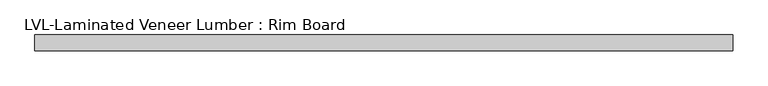
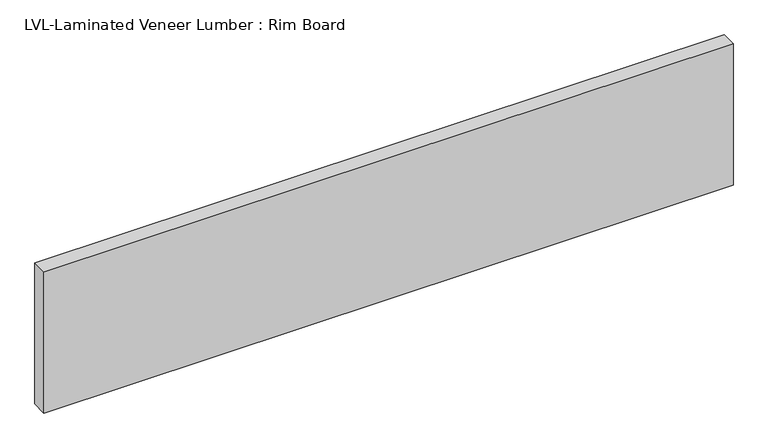
"""IFC4 building model written with IfcOpenShell, lengths in millimetres: beam geometry, LVL-Laminated Veneer Lumber : Rim Board."""

from ifc_helpers import new_model, si_unit, frame, origin, place, context, project, spatial, polyline, outline, extrude, source, transform, mapped, element, save


def lvl_laminated_veneer_lumber_rim_board_f89b900f(model_context):
    return source(origin(), model_context, "Body", "SweptSolid", [
        extrude(outline(polyline([(695.325, 15.875), (695.325, -15.875), (-695.325, -15.875), (-695.325, 15.875), (695.325, 15.875)])), frame((0.0, 0.0, -150.8125), z_axis=(0.0, 0.0, 1.0), x_axis=(1.0, 0.0, 0.0)), (0.0, 0.0, 1.0), 301.625),
    ])


if __name__ == "__main__":
    model = new_model("IFC4")
    model_context = context("Model", 3, world=origin())
    ifc_project = project(units=[si_unit("LENGTHUNIT", "METRE", prefix="MILLI")], contexts=[model_context])
    site = spatial("IfcSite", under=ifc_project)
    building = spatial("IfcBuilding", under=site)
    placement = place(None, origin())
    lvl_laminated_veneer_lumber_rim_board_shape = lvl_laminated_veneer_lumber_rim_board_f89b900f(model_context)
    element("IfcBeam", 1, ObjectType="LVL-Laminated Veneer Lumber : Rim Board", at=placement, inside=building, context=model_context, shape_type="MappedRepresentation", body=[
        mapped(lvl_laminated_veneer_lumber_rim_board_shape, transform((0.0, 0.0, 0.0), x_axis=(1.0, 0.0, 0.0), y_axis=(0.0, 1.0, 0.0), z_axis=(0.0, 0.0, 1.0))),
    ])
    save(model, "model.ifc")

# Revit data of these elements
# Type "LVL-Laminated Veneer Lumber : Rim Board"
#   Assembly Code = "B10"
#   Cost = 4.6
#   Length [instance default] = 5' - 0"
#   b = 0' - 1 1/4"
#   d = 0' - 11 7/8"
#   Structural Material [instance default] = Softwood, Lumber
# Element 1 (IfcBeam, "LVL-Laminated Veneer Lumber : Rim Board")
#   Structural Material = Douglas Fir #2
#   Materials on its faces: "Douglas Fir #2"
# Materials
#   "Softwood, Lumber": class "Wood", colour RGB 223 192 134, transparency 0, Description = "Pinus Echinata", Cost = 0
#   "Douglas Fir #2": class "Wood", colour RGB 223 192 134, transparency 0, Description = "Pinus Echinata", Cost = 0
